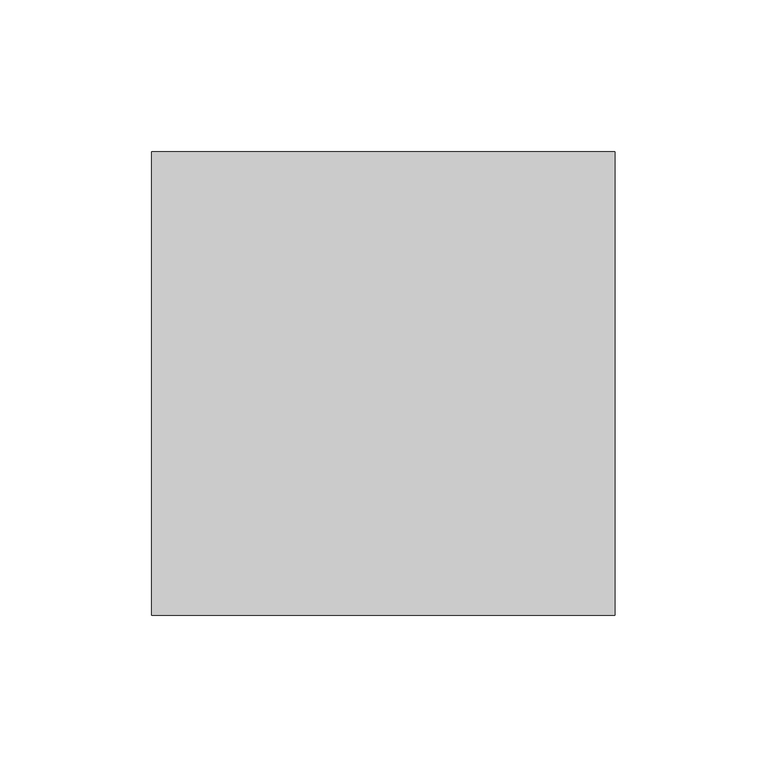
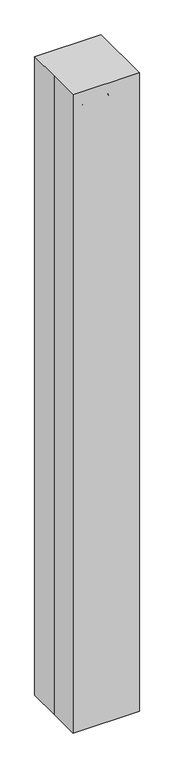
"""IFC4 building model written with IfcOpenShell, lengths in millimetres: proxy geometry, M8513 - Duodenoscope, Fiberoptic, Therapeutic : M8513 - Duodenoscope, Fiberoptic, Therapeutic."""

from ifc_helpers import new_model, si_unit, point, frame, origin, origin_with_axes, place, context, project, spatial, polyline, circle_curve, ellipse_curve, trimmed, outline, extrude, source, transform, mapped, element, save
from ifc_brep_helpers import plane_surface, cylinder_surface, revolved_surface, advanced_brep


def specialty_equipment_258c5ad5(model_context):
    return source(origin(), model_context, "Body", "SolidModel", [
        extrude(outline(polyline([(-12.7, -34.925), (-50.8, -34.925), (-50.8, -9.525), (-12.7, -9.525), (-12.7, -34.925)])), origin_with_axes(), (0.0, 0.0, 1.0), 101.6),
        advanced_brep(
        [(-25.4, -22.225, 101.6), (-38.1, -22.225, 101.6), (25.4, -22.225, 0.0), (38.1, -22.225, 0.0), (-25.4, -22.225, 1466.85), (-38.1, -22.225, 1466.85), (38.1, -22.225, 1466.85), (25.4, -22.225, 1466.85)],
        [
            (0, 1, circle_curve(frame((-31.75, -22.225, 101.6), z_axis=(0.0, 0.0, -1.0), x_axis=(-1.0, 0.0, 0.0)), 6.35)),
            (1, 0, circle_curve(frame((-31.75, -22.225, 101.6), z_axis=(0.0, 0.0, -1.0), x_axis=(-1.0, 0.0, 0.0)), 6.35)),
            (2, 3, circle_curve(frame((31.75, -22.225, 0.0), z_axis=(0.0, 0.0, -1.0), x_axis=(1.0, 0.0, 0.0)), 6.35)),
            (3, 2, circle_curve(frame((31.75, -22.225, 0.0), z_axis=(0.0, 0.0, -1.0), x_axis=(1.0, 0.0, 0.0)), 6.35)),
            (0, 4),
            (4, 5, circle_curve(frame((-31.75, -22.225, 1466.85), z_axis=(0.0, 0.0, -1.0), x_axis=(-1.0, 0.0, 0.0)), 6.35)),
            (5, 1),
            (5, 4, circle_curve(frame((-31.75, -22.225, 1466.85), z_axis=(0.0, 0.0, -1.0), x_axis=(-1.0, 0.0, 0.0)), 6.35)),
            (6, 7, circle_curve(frame((31.75, -22.225, 1466.85), z_axis=(0.0, 0.0, -1.0), x_axis=(1.0, 0.0, 0.0)), 6.35)),
            (7, 2),
            (3, 6),
            (7, 6, circle_curve(frame((31.75, -22.225, 1466.85), z_axis=(0.0, 0.0, -1.0), x_axis=(1.0, 0.0, 0.0)), 6.35)),
            (6, 5, circle_curve(frame((0.0, -22.225, 1466.85), z_axis=(0.0, -1.0, 0.0), x_axis=(-1.0, 0.0, 0.0)), 38.1)),
            (4, 7, circle_curve(frame((0.0, -22.225, 1466.85), z_axis=(0.0, 1.0, 0.0), x_axis=(-1.0, 0.0, 0.0)), 25.4)),
        ],
        [
            plane_surface(frame((-31.75, 41.275, 101.6), z_axis=(0.0, 0.0, -1.0), x_axis=(0.0, -1.0, 0.0))),
            plane_surface(frame((31.75, 41.275, 0.0), z_axis=(0.0, 0.0, -1.0), x_axis=(0.0, -1.0, 0.0))),
            cylinder_surface(frame((-31.75, -22.225, 101.6), z_axis=(0.0, 0.0, -1.0), x_axis=(-1.0, 0.0, 0.0)), 6.35),
            cylinder_surface(frame((31.75, -22.225, 1466.85), z_axis=(0.0, 0.0, 1.0), x_axis=(1.0, 0.0, 0.0)), 6.35),
            revolved_surface(trimmed(ellipse_curve(frame((-31.75, -22.225, 1466.85), z_axis=(0.0, 0.0, -1.0), x_axis=(-1.0, 0.0, 0.0)), 6.35, 6.35), [point((-25.4, -22.225, 1466.85))], [point((-38.1, -22.225, 1466.85))], True, "CARTESIAN"), (0.0, 41.275, 1466.85), (0.0, 1.0, 0.0)),
            revolved_surface(trimmed(ellipse_curve(frame((-31.75, -22.225, 1466.85), z_axis=(0.0, 0.0, -1.0), x_axis=(-1.0, 0.0, 0.0)), 6.35, 6.35), [point((-38.1, -22.225, 1466.85))], [point((-25.4, -22.225, 1466.85))], True, "CARTESIAN"), (0.0, 41.275, 1466.85), (0.0, 1.0, 0.0)),
        ],
        [
            (0, [[1, 2]]),
            (1, [[3, 4]]),
            (2, [[-1, 5, 6, 7]]),
            (2, [[-2, -7, 8, -5]]),
            (3, [[9, 10, -4, 11]]),
            (3, [[12, -11, -3, -10]]),
            (4, [[13, -6, 14, -9]]),
            (5, [[-14, -8, -13, -12]]),
        ],
    ),
        extrude(outline(polyline([(-76.2, 76.2), (76.2, 76.2), (76.2, -76.2), (-76.2, -76.2), (-76.2, 0.0), (-76.2, 76.2)])), origin_with_axes(), (0.0, 0.0, 1.0), 1549.4),
    ])


if __name__ == "__main__":
    model = new_model("IFC4")
    model_context = context("Model", 3, world=origin())
    ifc_project = project(units=[si_unit("LENGTHUNIT", "METRE", prefix="MILLI")], contexts=[model_context])
    site = spatial("IfcSite", under=ifc_project)
    building = spatial("IfcBuilding", under=site)
    placement = place(None, origin())
    specialty_equipment_shape = specialty_equipment_258c5ad5(model_context)
    element("IfcBuildingElementProxy", 1, Name="M8513 - Duodenoscope, Fiberoptic, Therapeutic : M8513 - Duodenoscope, Fiberoptic, Therapeutic", ObjectType="M8513 - Duodenoscope, Fiberoptic, Therapeutic : M8513 - Duodenoscope, Fiberoptic, Therapeutic", at=placement, inside=building, context=model_context, shape_type="MappedRepresentation", body=[
        mapped(specialty_equipment_shape, transform((0.0, 0.0, 0.0), x_axis=(1.0, 0.0, 0.0), y_axis=(0.0, 1.0, 0.0), z_axis=(0.0, 0.0, 1.0))),
    ])
    save(model, "model.ifc")

# Revit data of these elements
# Type "M8513 - Duodenoscope, Fiberoptic, Therapeutic : M8513 - Duodenoscope, Fiberoptic, Therapeutic"
#   Watts2 = "0"
#   Watts1 = "0"
#   Unit_Issue = "EA"
#   UTIL_6_Misc = "-"
#   UTIL_5_NonMedGas = "-"
#   UTIL_4_MiscGas = "-"
#   UTIL_3_MedGas = "-"
#   UTIL_2_Elec = "-"
#   UTIL_1_WaterDrain = "-"
#   Nomenclature = "Duodenoscope, Fiberoptic, Therapeutic"
#   NSN = "6515"
#   Location [instance default] = ""
#   JSN = "M8513"
#   Fund_Source_VA = "-"
#   Fund_Source_Navy = "-"
#   Fund_Source_Army = "-"
#   Fund_Source_AF = "-"
#   ELEC_Volts2 = "0"
#   ELEC_Volts1 = "0"
#   ELEC_Phase2 = "0"
#   ELEC_Phase1 = "0"
#   ELEC_HertzSwitch = "0"
#   ELEC_HertzDependent = "0"
#   ELEC_Hertz = "0"
#   ELEC_Amps2 = "0"
#   ELEC_Amps1 = "0"
#   DetailDescription = "Flexible fiberoptic duodenoscope. This scope is designed for duodenal exploration, volume washings, biopsy or tissue removal and suctioning. Unit consists of a thin flexible casing with a suction adapter, an instrument channel, an air/water channel, a light guide, an objective lens with an optical image fiber cluster, a forceps raiser, an eyepiece and a cable for connection to a light source. Casings and instrument channels can have varying dimensions depending on duodenoscope design and intended procedure."
#   CAT_VA = "C"
#   CAT_Navy = "C"
#   CAT_IHS = "-"
#   CAT_Army = "C"
#   CAT_AF = "C"
#   BTUperhour = "0"
#   Weight_IP = 10
#   DIM_Width_IP = 0' - 6"
#   DIM_Height_IP = 0' - 6"
#   DIM_Depth_IP = 5' - 1"
# Element 1 (IfcBuildingElementProxy, "M8513 - Duodenoscope, Fiberoptic, Therapeutic : M8513 - Duodenoscope, Fiberoptic, Therapeutic")
#   Location = "TREE1"
#   Materials on its faces: "EquipSpace"
# Materials
#   "EquipSpace": class "Miscellaneous", colour RGB 221 217 195, transparency 0.5
